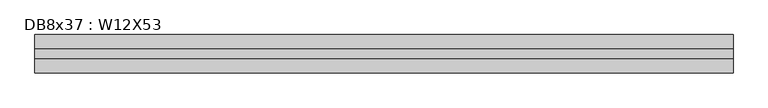
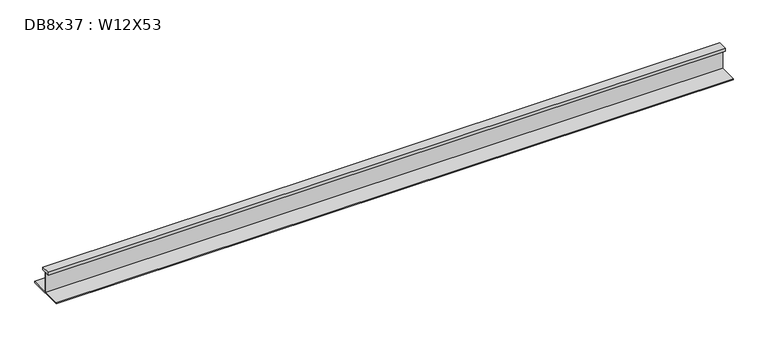
"""IFC4 building model written with IfcOpenShell, lengths in millimetres: beam geometry, DB8x37 : W12X53."""

from ifc_helpers import new_model, si_unit, frame, origin, place, context, project, spatial, polyline, outline, extrude, source, transform, mapped, element, save


def db8x37_w12x53_32b51aad(model_context):
    return source(origin(), model_context, "Body", "SweptSolid", [
        extrude(outline(polyline([(38.1, 145.415), (38.1, 120.015), (2.921, 120.015), (2.921, -48.4505), (152.4, -48.4505), (152.4, -58.1025), (-152.4, -58.1025), (-152.4, -48.4505), (-2.921, -48.4505), (-2.921, 120.015), (-38.1, 120.015), (-38.1, 145.415), (38.1, 145.415)])), frame((-2705.1, 0.0, 0.0), z_axis=(1.0, 0.0, 0.0), x_axis=(0.0, 1.0, 0.0)), (0.0, 0.0, 1.0), 5537.1999994),
    ])


if __name__ == "__main__":
    model = new_model("IFC4")
    model_context = context("Model", 3, world=origin())
    ifc_project = project(units=[si_unit("LENGTHUNIT", "METRE", prefix="MILLI")], contexts=[model_context])
    site = spatial("IfcSite", under=ifc_project)
    building = spatial("IfcBuilding", under=site)
    placement = place(None, origin())
    db8x37_w12x53_shape = db8x37_w12x53_32b51aad(model_context)
    element("IfcBeam", 1, ObjectType="DB8x37 : W12X53", at=placement, inside=building, context=model_context, shape_type="MappedRepresentation", body=[
        mapped(db8x37_w12x53_shape, transform((0.0, 0.0, 0.0), x_axis=(1.0, 0.0, 0.0), y_axis=(0.0, 1.0, 0.0), z_axis=(0.0, 0.0, 1.0))),
    ])
    save(model, "model.ifc")

# Revit data of these elements
# Type "DB8x37 : W12X53"
#   Assembly Code = "B10"
#   W = 53
#   Length [instance default] = 5' - 0"
#   bf = 0' - 10"
#   d = 1' - 0.1"
#   k = 0' - 1 3/8"
#   k2 = 0' - 0.8"
#   tf = 0' - 0.575"
#   tw = 0' - 0.345"
#   A = 0.108333 SF
#   Structural Material [instance default] = Steel ASTM A992
# Element 1 (IfcBeam, "DB8x37 : W12X53")
#   Materials on its faces: "Steel ASTM A992"
# Materials
#   "Steel ASTM A992": class "Metal", colour RGB 199 199 199, transparency 0, Description = "Structural steel 50ksi", Cost = 0
